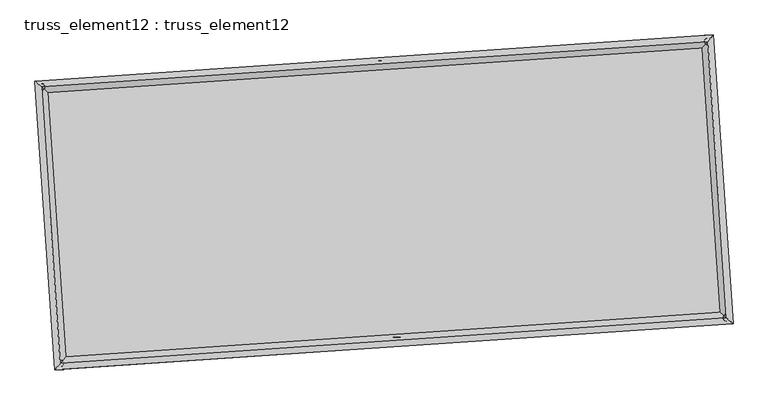
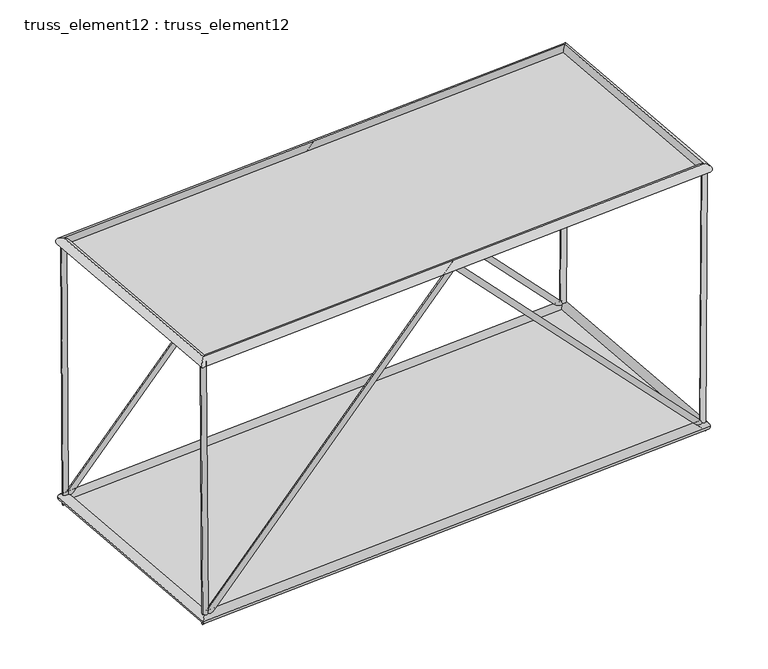
"""IFC4 building model written with IfcOpenShell, lengths in millimetres: plate geometry, truss_element12 : truss_element12."""

from ifc_helpers import new_model, si_unit, frame, origin, origin_with_axes, place, context, project, spatial, polyline, circle_curve, ellipse_curve, outline, extrude, source, transform, mapped, element, save
from ifc_brep_helpers import plane_surface, cylinder_surface, advanced_brep


def truss_element12_truss_element12_52c30542(model_context):
    return source(origin(), model_context, "Body", "SolidModel", [
        advanced_brep(
        [(-3697.2399315, 2274.0216798, 5000.2182213), (-3796.341209, 2260.6605634, 4999.5721856), (-3665.7376222, 2276.1697025, 123.3684654), (-3763.2492606, 2262.9169776, -123.3684654), (1063.9678225, 2598.6703375, 5072.0167467), (1064.4123159, 2592.0968689, 4927.7704358), (5793.1885788, 2921.1379234, 123.3649609), (5891.5723982, 2921.2425651, -123.3649609), (5825.1718993, 2923.3187444, 5000.2199286), (5925.1695178, 2923.533425, 4999.5640296)],
        [
            (0, 1, circle_curve(frame((-3746.7905702, 2267.3411216, 4999.8952035), z_axis=(-0.006459425759977356, -0.00044044368800008225, 0.9999790406944584), x_axis=(-0.1336112082599859, 0.9910337345765261, -0.0004265660679954251)), 50.0)),
            (1, 0, circle_curve(frame((-3746.7905702, 2267.3411216, 4999.8952035), z_axis=(-0.006459425759977356, -0.00044044368800008225, 0.9999790406944584), x_axis=(-0.1336112082599859, 0.9910337345765261, -0.0004265660679954251)), 50.0)),
            (0, 2),
            (2, 3, ellipse_curve(frame((-3714.4934414, 2269.54334, 0.0), z_axis=(-0.9269817502517961, -0.06320736176214563, 0.36974269988626707), x_axis=(0.3688861524964249, 0.025152944471183856, 0.9291341861544079)), 133.0670008, 50.0)),
            (3, 1),
            (3, 2, ellipse_curve(frame((-3714.4934414, 2269.54334, 0.0), z_axis=(-0.9269817502517961, -0.06320736176214563, 0.36974269988626707), x_axis=(0.3688861524964249, 0.025152944471183856, 0.9291341861544079)), 133.0670008, 50.0)),
            (2, 4),
            (4, 5, ellipse_curve(frame((1064.1900692, 2595.3836032, 4999.8935913), z_axis=(-0.9976833957434986, -0.06802823820610797, 2.5773915170605543e-05), x_axis=(-2.5714207217699398e-05, -1.7533540379466907e-06, -0.9999999996678528)), 72.2802032, 50.0)),
            (5, 3),
            (5, 4, ellipse_curve(frame((1064.1900692, 2595.3836032, 4999.8935913), z_axis=(-0.9976833957434986, -0.06802823820610797, 2.5773915170605543e-05), x_axis=(-2.5714207217699398e-05, -1.7533540379466907e-06, -0.9999999996678528)), 72.2802032, 50.0)),
            (4, 6),
            (6, 7, ellipse_curve(frame((5842.3804885, 2921.1902443, 0.0), z_axis=(-0.9270094873495353, -0.06320925304939957, -0.36967282925972333), x_axis=(-0.3688164437324487, -0.02514819129556234, 0.9291619876572177)), 133.0592395, 50.0)),
            (7, 5),
            (7, 6, ellipse_curve(frame((5842.3804885, 2921.1902443, 0.0), z_axis=(-0.9270094873495353, -0.06320925304939957, -0.36967282925972333), x_axis=(-0.3688164437324487, -0.02514819129556234, 0.9291619876572177)), 133.0592395, 50.0)),
            (8, 9, circle_curve(frame((5875.1707086, 2923.4260847, 4999.8919791), z_axis=(0.0065580440171246965, 0.00044716809206525154, 0.9999783958163131), x_axis=(-0.0021496921144927646, 0.9999975956304801, -0.00043307859770738705)), 50.0)),
            (9, 8, circle_curve(frame((5875.1707086, 2923.4260847, 4999.8919791), z_axis=(0.0065580440171246965, 0.00044716809206525154, 0.9999783958163131), x_axis=(-0.0021496921144927646, 0.9999975956304801, -0.00043307859770738705)), 50.0)),
            (6, 8),
            (9, 7),
        ],
        [
            plane_surface(frame((-3746.7905702, 2317.3411168, 4999.9172261), z_axis=(-0.006459425759978043, -0.0004404436880029011, 0.9999790406944582), x_axis=(0.9999791376918077, -2.8450726592410543e-06, 0.006459425133417794))),
            cylinder_surface(frame((-3746.7905702, 2267.3411216, 4999.8952035), z_axis=(-0.006459425759977354, -0.00044044368800008214, 0.9999790406944582), x_axis=(-0.1336112082599859, 0.9910337345765261, -0.0004265660679954251)), 50.0),
            cylinder_surface(frame((-3714.4934414, 2269.54334, 0.0), z_axis=(-0.6901683966914209, -0.0470599593946937, -0.7221169880498335), x_axis=(-0.020414121785071758, 0.9987522136008405, -0.04557718134291885)), 50.0),
            cylinder_surface(frame((1064.1900692, 2595.3836032, 4999.8935913), z_axis=(-0.6901312584427504, -0.04705742707869742, 0.7221526463822996), x_axis=(-0.1153490800992824, 0.9922789596749564, -0.04557472881582181)), 50.0),
            plane_surface(frame((5875.1707086, 2873.4260897, 4999.914338), z_axis=(0.0065580440171256905, 0.0004471680920647648, 0.9999783958163133), x_axis=(0.9999784957981195, -2.932611094408339e-06, -0.006558043361426502))),
            cylinder_surface(frame((5842.3804885, 2921.1902443, 0.0), z_axis=(-0.0065580440171246965, -0.00044716809206525154, -0.9999783958163131), x_axis=(-0.0021496921144927646, 0.9999975956304801, -0.00043307859770738705)), 50.0),
        ],
        [
            (0, [[1, 2]]),
            (1, [[-1, 3, 4, 5]]),
            (1, [[-2, -5, 6, -3]]),
            (2, [[-4, 7, 8, 9]]),
            (2, [[-6, -9, 10, -7]]),
            (3, [[-8, 11, 12, 13]]),
            (3, [[-10, -13, 14, -11]]),
            (4, [[15, 16]]),
            (5, [[-12, 17, -16, 18]]),
            (5, [[-14, -18, -15, -17]]),
        ],
    ),
        advanced_brep(
        [(-3425.1269785, -1716.7119045, 5000.2182213), (-3524.2282561, -1730.0730209, 4999.5721856), (-3393.6246693, -1714.5638818, 123.3684654), (-3491.1363077, -1727.8166067, -123.3684654), (1336.0807754, -1392.0632468, 5072.0167467), (1336.5252688, -1398.6367154, 4927.7704358), (6065.3015317, -1069.5956609, 123.3649609), (6163.6853511, -1069.4910192, -123.3649609), (6097.2848522, -1067.4148399, 5000.2199286), (6197.2824708, -1067.2001593, 4999.5640296)],
        [
            (0, 1, circle_curve(frame((-3474.6776173, -1723.3924627, 4999.8952035), z_axis=(-0.006459425759977131, -0.0004404436880000592, 0.9999790406944584), x_axis=(-0.1336112082599859, 0.9910337345765261, -0.00042656606799541797)), 50.0)),
            (1, 0, circle_curve(frame((-3474.6776173, -1723.3924627, 4999.8952035), z_axis=(-0.006459425759977131, -0.0004404436880000592, 0.9999790406944584), x_axis=(-0.1336112082599859, 0.9910337345765261, -0.00042656606799541797)), 50.0)),
            (0, 2),
            (2, 3, ellipse_curve(frame((-3442.3804885, -1721.1902443, 0.0), z_axis=(-0.9269817502517953, -0.06320736176214553, 0.36974269988626884), x_axis=(0.3688861524964267, 0.02515294447118397, 0.9291341861544073)), 133.0670008, 50.0)),
            (3, 1),
            (3, 2, ellipse_curve(frame((-3442.3804885, -1721.1902443, 0.0), z_axis=(-0.9269817502517953, -0.06320736176214553, 0.36974269988626884), x_axis=(0.3688861524964267, 0.02515294447118397, 0.9291341861544073)), 133.0670008, 50.0)),
            (2, 4),
            (4, 5, ellipse_curve(frame((1336.3030221, -1395.3499811, 4999.8935913), z_axis=(-0.9976833957434985, -0.06802823820610795, 2.577391517253143e-05), x_axis=(-2.5714207220005564e-05, -1.7533540380716083e-06, -0.9999999996678525)), 72.2802032, 50.0)),
            (5, 3),
            (5, 4, ellipse_curve(frame((1336.3030221, -1395.3499811, 4999.8935913), z_axis=(-0.9976833957434985, -0.06802823820610795, 2.577391517253143e-05), x_axis=(-2.5714207220005564e-05, -1.7533540380716083e-06, -0.9999999996678525)), 72.2802032, 50.0)),
            (4, 6),
            (6, 7, ellipse_curve(frame((6114.4934414, -1069.54334, 0.0), z_axis=(-0.9270094873495354, -0.06320925304939953, -0.36967282925972317), x_axis=(-0.36881644373244843, -0.025148191295562353, 0.9291619876572176)), 133.0592395, 50.0)),
            (7, 5),
            (7, 6, ellipse_curve(frame((6114.4934414, -1069.54334, 0.0), z_axis=(-0.9270094873495354, -0.06320925304939953, -0.36967282925972317), x_axis=(-0.36881644373244843, -0.025148191295562353, 0.9291619876572176)), 133.0592395, 50.0)),
            (8, 9, circle_curve(frame((6147.2836615, -1067.3074996, 4999.8919791), z_axis=(0.006558044017124805, 0.00044716809206521056, 0.9999783958163131), x_axis=(-0.0021496921144928067, 0.9999975956304801, -0.0004330785977073455)), 50.0)),
            (9, 8, circle_curve(frame((6147.2836615, -1067.3074996, 4999.8919791), z_axis=(0.006558044017124805, 0.00044716809206521056, 0.9999783958163131), x_axis=(-0.0021496921144928067, 0.9999975956304801, -0.0004330785977073455)), 50.0)),
            (6, 8),
            (9, 7),
        ],
        [
            plane_surface(frame((-3474.6776173, -1673.3924675, 4999.9172261), z_axis=(-0.006459425759978043, -0.0004404436880029083, 0.9999790406944582), x_axis=(0.9999791376918077, -2.8450726592410543e-06, 0.006459425133417794))),
            cylinder_surface(frame((-3474.6776173, -1723.3924627, 4999.8952035), z_axis=(-0.006459425759977129, -0.0004404436880000591, 0.9999790406944582), x_axis=(-0.1336112082599859, 0.9910337345765261, -0.00042656606799541797)), 50.0),
            cylinder_surface(frame((-3442.3804885, -1721.1902443, 0.0), z_axis=(-0.6901683966914234, -0.04705995939469384, -0.722116988049831), x_axis=(-0.020414121785071914, 0.9987522136008405, -0.04557718134291897)), 50.0),
            cylinder_surface(frame((1336.3030221, -1395.3499811, 4999.8935913), z_axis=(-0.6901312584427504, -0.04705742707869744, 0.7221526463823), x_axis=(-0.11534908009928244, 0.9922789596749565, -0.045574728815821794)), 50.0),
            plane_surface(frame((6147.2836615, -1117.3074946, 4999.914338), z_axis=(0.00655804401712569, 0.0004471680920647726, 0.9999783958163132), x_axis=(0.9999784957981195, -2.932611094408339e-06, -0.006558043361426502))),
            cylinder_surface(frame((6114.4934414, -1069.54334, 0.0), z_axis=(-0.006558044017124805, -0.00044716809206521056, -0.9999783958163131), x_axis=(-0.0021496921144928067, 0.9999975956304801, -0.0004330785977073455)), 50.0),
        ],
        [
            (0, [[1, 2]]),
            (1, [[-1, 3, 4, 5]]),
            (1, [[-2, -5, 6, -3]]),
            (2, [[-4, 7, 8, 9]]),
            (2, [[-6, -9, 10, -7]]),
            (3, [[-8, 11, 12, 13]]),
            (3, [[-10, -13, 14, -11]]),
            (4, [[15, 16]]),
            (5, [[-12, 17, -16, 18]]),
            (5, [[-14, -18, -15, -17]]),
        ],
    ),
        advanced_brep(
        [(-3474.6784688, -1723.3934064, 4909.8952035), (-3474.6767658, -1723.391519, 5089.8952035), (-3746.7895985, 2267.3403022, 5089.8952035), (-3746.7915419, 2267.341941, 4909.8952035), (5875.1699172, 2923.4251451, 5089.8919791), (5875.1715, 2923.4270243, 4909.8919791), (6147.2827499, -1067.3066761, 5089.8919791), (6147.2845731, -1067.3083231, 4909.8919791)],
        [
            (0, 1, ellipse_curve(frame((-3474.6776173, -1723.3924627, 4999.8952035), z_axis=(-0.7535719234054118, 0.6573654662780912, 2.3640779700271338e-07), x_axis=(-0.6573654662780491, -0.7535719234054485, 2.3640780925401256e-07)), 127.2792206, 90.0)),
            (1, 2),
            (2, 3, ellipse_curve(frame((-3746.7905702, 2267.3411216, 4999.8952035), z_axis=(-0.6573654662780489, -0.7535719234054485, 2.364078067134504e-07), x_axis=(0.7535719234054117, -0.6573654662780912, -2.3640779446215126e-07)), 127.2792206, 90.0)),
            (3, 0),
            (1, 0, ellipse_curve(frame((-3474.6776173, -1723.3924627, 4999.8952035), z_axis=(-0.7535719234054118, 0.6573654662780912, 2.3640779700271338e-07), x_axis=(-0.6573654662780491, -0.7535719234054485, 2.3640780925401256e-07)), 127.2792206, 90.0)),
            (3, 2, ellipse_curve(frame((-3746.7905702, 2267.3411216, 4999.8952035), z_axis=(-0.6573654662780489, -0.7535719234054485, 2.364078067134504e-07), x_axis=(0.7535719234054117, -0.6573654662780912, -2.3640779446215126e-07)), 127.2792206, 90.0)),
            (2, 4),
            (4, 5, ellipse_curve(frame((5875.1707086, 2923.4260847, 4999.8919791), z_axis=(-0.7535719234054148, 0.6573654662780879, 2.3640780058782646e-07), x_axis=(-0.6573654662780456, -0.7535719234054514, 2.3640780058777527e-07)), 127.2792206, 90.0)),
            (5, 3),
            (5, 4, ellipse_curve(frame((5875.1707086, 2923.4260847, 4999.8919791), z_axis=(-0.7535719234054148, 0.6573654662780879, 2.3640780058782646e-07), x_axis=(-0.6573654662780456, -0.7535719234054514, 2.3640780058777527e-07)), 127.2792206, 90.0)),
            (4, 6),
            (6, 7, ellipse_curve(frame((6147.2836615, -1067.3074996, 4999.8919791), z_axis=(0.6573654662780457, 0.7535719234054514, -2.3640780312833733e-07), x_axis=(-0.7535719234054146, 0.6573654662780879, 2.3640780312838847e-07)), 127.2792206, 90.0)),
            (7, 5),
            (7, 6, ellipse_curve(frame((6147.2836615, -1067.3074996, 4999.8919791), z_axis=(0.6573654662780457, 0.7535719234054514, -2.3640780312833733e-07), x_axis=(-0.7535719234054146, 0.6573654662780879, 2.3640780312838847e-07)), 127.2792206, 90.0)),
            (6, 1),
            (0, 7),
        ],
        [
            cylinder_surface(frame((-3474.6776173, -1723.3924627, 4999.8952035), z_axis=(0.06802823822868682, -0.9976833960748777, 0.0), x_axis=(-0.9976833960234641, -0.06802823822518114, 1.0152132486798217e-05)), 90.0),
            cylinder_surface(frame((-3746.7905702, 2267.3411216, 4999.8952035), z_axis=(-0.9976833960748211, -0.06802823822869182, 3.3433111784206217e-07), x_axis=(-0.06802823822214224, 0.9976833960270173, 9.81780136030937e-06)), 90.0),
            cylinder_surface(frame((5875.1707086, 2923.4260847, 4999.8919791), z_axis=(-0.06802823822869526, 0.9976833960748771, 0.0), x_axis=(0.9976833960300131, 0.06802823822563615, 9.483470242483464e-06)), 90.0),
            cylinder_surface(frame((6147.2836615, -1067.3074996, 4999.8919791), z_axis=(0.9976833960748215, 0.0680282382286917, -3.343311214349595e-07), x_axis=(0.06802823822869168, -0.9976833960265709, 9.81780136390235e-06)), 90.0),
        ],
        [
            (0, [[1, 2, 3, 4]]),
            (0, [[5, -4, 6, -2]]),
            (1, [[-3, 7, 8, 9]]),
            (1, [[-6, -9, 10, -7]]),
            (2, [[-8, 11, 12, 13]]),
            (2, [[-10, -13, 14, -11]]),
            (3, [[-12, 15, -1, 16]]),
            (3, [[-14, -16, -5, -15]]),
        ],
    ),
        advanced_brep(
        [(-3358.7115243, -1625.2761972, 0.0), (-3526.0494527, -1817.1042913, 0.0), (-3810.4074885, 2353.2123043, 0.0), (-3618.5793943, 2185.8743758, 0.0), (5926.0494527, 3017.1042913, 0.0), (5758.7115243, 2825.2761972, 0.0), (6210.4074885, -1153.2123043, 0.0), (6018.5793943, -985.8743758, 0.0)],
        [
            (0, 1, ellipse_curve(frame((-3442.3804885, -1721.1902443, 0.0), z_axis=(-0.7535719234054562, 0.6573654662780828, 0.0), x_axis=(-0.6573654662780827, -0.7535719234054563, 0.0)), 127.2792206, 90.0)),
            (1, 2),
            (2, 3, ellipse_curve(frame((-3714.4934414, 2269.54334, 0.0), z_axis=(-0.6573654662780828, -0.7535719234054561, 0.0), x_axis=(0.753571923405456, -0.6573654662780831, 0.0)), 127.2792206, 90.0)),
            (3, 0),
            (1, 0, ellipse_curve(frame((-3442.3804885, -1721.1902443, 0.0), z_axis=(-0.7535719234054562, 0.6573654662780828, 0.0), x_axis=(-0.6573654662780827, -0.7535719234054563, 0.0)), 127.2792206, 90.0)),
            (3, 2, ellipse_curve(frame((-3714.4934414, 2269.54334, 0.0), z_axis=(-0.6573654662780828, -0.7535719234054561, 0.0), x_axis=(0.753571923405456, -0.6573654662780831, 0.0)), 127.2792206, 90.0)),
            (2, 4),
            (4, 5, ellipse_curve(frame((5842.3804885, 2921.1902443, 0.0), z_axis=(-0.7535719234054591, 0.6573654662780796, 0.0), x_axis=(-0.6573654662780796, -0.7535719234054591, 0.0)), 127.2792206, 90.0)),
            (5, 3),
            (5, 4, ellipse_curve(frame((5842.3804885, 2921.1902443, 0.0), z_axis=(-0.7535719234054591, 0.6573654662780796, 0.0), x_axis=(-0.6573654662780796, -0.7535719234054591, 0.0)), 127.2792206, 90.0)),
            (4, 6),
            (6, 7, ellipse_curve(frame((6114.4934414, -1069.54334, 0.0), z_axis=(0.6573654662780796, 0.7535719234054591, 0.0), x_axis=(-0.7535719234054592, 0.6573654662780793, 0.0)), 127.2792206, 90.0)),
            (7, 5),
            (7, 6, ellipse_curve(frame((6114.4934414, -1069.54334, 0.0), z_axis=(0.6573654662780796, 0.7535719234054591, 0.0), x_axis=(-0.7535719234054592, 0.6573654662780793, 0.0)), 127.2792206, 90.0)),
            (6, 1),
            (0, 7),
        ],
        [
            cylinder_surface(frame((-3442.3804885, -1721.1902443, 0.0), z_axis=(0.06802823822869401, -0.9976833960748771, 0.0), x_axis=(-0.9976833960748771, -0.06802823822869401, 0.0)), 90.0),
            cylinder_surface(frame((-3714.4934414, 2269.54334, 0.0), z_axis=(-0.9976833960748764, -0.06802823822870314, 0.0), x_axis=(-0.06802823822870314, 0.9976833960748764, 0.0)), 90.0),
            cylinder_surface(frame((5842.3804885, 2921.1902443, 0.0), z_axis=(-0.06802823822870271, 0.9976833960748764, 0.0), x_axis=(0.9976833960748764, 0.06802823822870271, 0.0)), 90.0),
            cylinder_surface(frame((6114.4934414, -1069.54334, 0.0), z_axis=(0.9976833960748764, 0.06802823822870317, 0.0), x_axis=(0.06802823822870317, -0.9976833960748764, 0.0)), 90.0),
        ],
        [
            (0, [[1, 2, 3, 4]]),
            (0, [[5, -4, 6, -2]]),
            (1, [[-3, 7, 8, 9]]),
            (1, [[-6, -9, 10, -7]]),
            (2, [[-8, 11, 12, 13]]),
            (2, [[-10, -13, 14, -11]]),
            (3, [[-12, 15, -1, 16]]),
            (3, [[-14, -16, -5, -15]]),
        ],
    ),
        extrude(outline(polyline([(-3442.3804885, -1721.1902443), (-3714.4934414, 2269.54334), (5842.3804885, 2921.1902443), (6114.4934414, -1069.54334), (-3442.3804885, -1721.1902443)])), origin_with_axes(), (0.0, 0.0, 1.0), 20.0),
        extrude(outline(polyline([(-2000.0, 4822.1516548), (2000.0, 4822.1516548), (2000.0, -4822.1516549), (-2000.0, -4822.1516549), (-2000.0, 4822.1516548)])), frame((1200.2465456, 600.016811, 4999.8935913), z_axis=(3.3355660447281574e-07, 2.2743965574691364e-08, 0.9999999999999442), x_axis=(-0.06802823822869453, 0.9976833960748771, 0.0)), (0.0, 0.0, 1.0), 20.0),
    ])


if __name__ == "__main__":
    model = new_model("IFC4")
    model_context = context("Model", 3, world=origin())
    ifc_project = project(units=[si_unit("LENGTHUNIT", "METRE", prefix="MILLI")], contexts=[model_context])
    site = spatial("IfcSite", under=ifc_project)
    building = spatial("IfcBuilding", under=site)
    placement = place(None, origin())
    truss_element12_truss_element12_shape = truss_element12_truss_element12_52c30542(model_context)
    element("IfcPlate", 1, ObjectType="truss_element12 : truss_element12", at=placement, inside=building, context=model_context, shape_type="MappedRepresentation", body=[
        mapped(truss_element12_truss_element12_shape, transform((0.0, 0.0, 0.0), x_axis=(1.0, 0.0, 0.0), y_axis=(0.0, 1.0, 0.0), z_axis=(0.0, 0.0, 1.0))),
    ])
    save(model, "model.ifc")

# Revit data of these elements
# Type "truss_element12 : truss_element12"
#   steellbar1 = 90 mm
#   steelbar2 = 50 mm
#   offset1 = 5000 mm
#   M = Default Roof
# Element 1 (IfcPlate, "truss_element12 : truss_element12")
#   Materials on its faces: "Default Roof"
# Materials
#   "Default Roof": class "Miscellaneous", colour RGB 0 127 0, transparency 0, Comments = "Rendering appearance not upgraded Rendering appearance not upgraded ", Cost = 0
